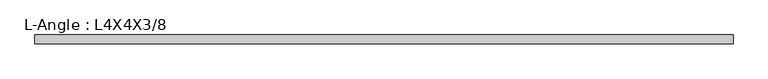
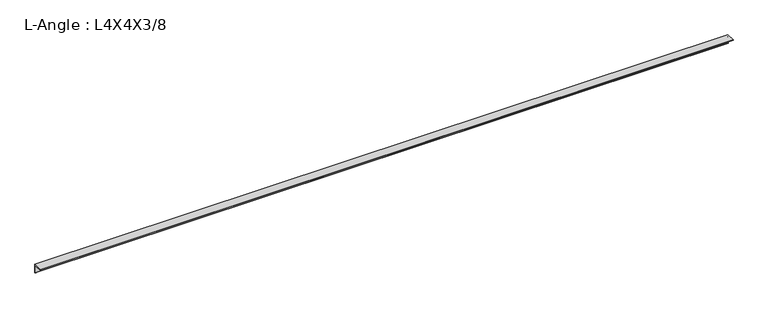
"""IFC4 building model written with IfcOpenShell, lengths in millimetres: beam geometry, L-Angle : L4X4X3/8."""

from ifc_helpers import new_model, si_unit, point, frame, frame_2d, origin, place, context, project, spatial, polyline, circle_curve, trimmed, segment, composite_curve, outline, extrude, source, transform, mapped, element, save


def l_angle_l4x4x3_8_334976ec(model_context):
    return source(origin(), model_context, "Body", "SweptSolid", [
        extrude(outline(composite_curve([segment(polyline([(28.702, 28.702), (28.702, -72.898)]), True, "CONTINUOUS"), segment(trimmed(circle_curve(frame_2d((28.702, -63.373)), 9.525), [point((28.702, -72.898))], [point((19.177, -63.373))], False, "CARTESIAN"), True, "CONTINUOUS"), segment(polyline([(19.177, -63.373), (19.177, 9.652)]), True, "CONTINUOUS"), segment(trimmed(circle_curve(frame_2d((9.652, 9.652)), 9.525), [point((19.177, 9.652))], [point((9.652, 19.177))], True, "CARTESIAN"), True, "CONTINUOUS"), segment(polyline([(9.652, 19.177), (-63.373, 19.177)]), True, "CONTINUOUS"), segment(trimmed(circle_curve(frame_2d((-63.373, 28.702)), 9.525), [point((-63.373, 19.177))], [point((-72.898, 28.702))], False, "CARTESIAN"), True, "CONTINUOUS"), segment(polyline([(-72.898, 28.702), (28.702, 28.702)]), True, "CONTINUOUS")], self_intersect=False)), frame((-3927.820956, 0.0, 0.0), z_axis=(1.0, 0.0, 0.0), x_axis=(0.0, 1.0, 0.0)), (0.0, 0.0, 1.0), 7938.0439602),
    ])


if __name__ == "__main__":
    model = new_model("IFC4")
    model_context = context("Model", 3, world=origin())
    ifc_project = project(units=[si_unit("LENGTHUNIT", "METRE", prefix="MILLI")], contexts=[model_context])
    site = spatial("IfcSite", under=ifc_project)
    building = spatial("IfcBuilding", under=site)
    placement = place(None, origin())
    l_angle_l4x4x3_8_shape = l_angle_l4x4x3_8_334976ec(model_context)
    element("IfcBeam", 1, ObjectType="L-Angle : L4X4X3/8", at=placement, inside=building, context=model_context, shape_type="MappedRepresentation", body=[
        mapped(l_angle_l4x4x3_8_shape, transform((0.0, 0.0, 0.0), x_axis=(1.0, 0.0, 0.0), y_axis=(0.0, 1.0, 0.0), z_axis=(0.0, 0.0, 1.0))),
    ])
    save(model, "model.ifc")

# Revit data of these elements
# Type "L-Angle : L4X4X3/8"
#   Assembly Code = "B10"
#   k = 0' - 0 3/4"
#   W = 9.8
#   Length [instance default] = 5' - 0"
#   b = 0' - 4"
#   d = 0' - 4"
#   t = 0' - 0 3/8"
#   x = 0' - 1.13"
#   y = 0' - 1.13"
#   A = 0.0198611 SF
#   Structural Material [instance default] = Steel ASTM A36
# Element 1 (IfcBeam, "L-Angle : L4X4X3/8")
#   Materials on its faces: "Steel ASTM A36"
# Materials
#   "Steel ASTM A36": class "Metal", colour RGB 199 199 199, transparency 0, Description = "Structural steel, ASTM A36 Grade B, mill finish", Cost = 0
